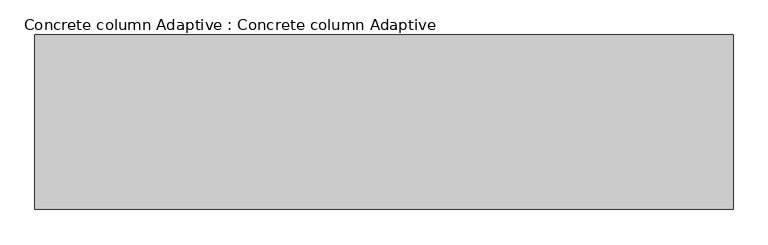
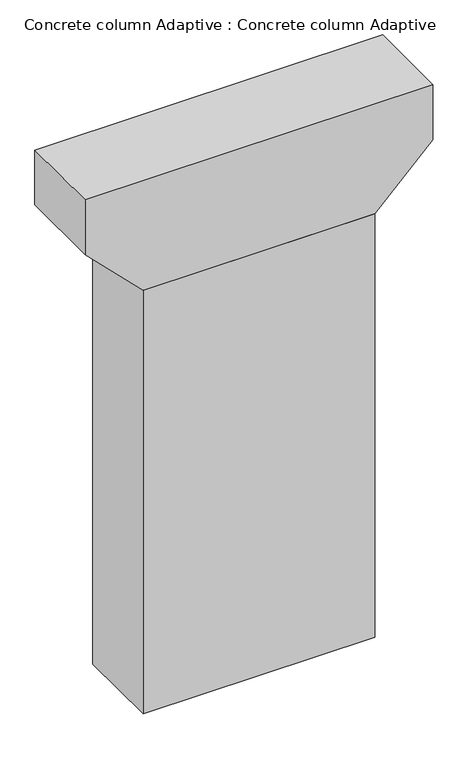
"""IFC4 building model written with IfcOpenShell, lengths in millimetres: proxy geometry, Concrete column Adaptive : Concrete column Adaptive."""

import ifcopenshell
import ifcopenshell.guid

model = None  # the IFC model being written
_history = None  # IfcOwnerHistory: only IFC2X3 demands one
_inside = {}  # id of a spatial element -> (the spatial element, [elements in it])
_under = {}  # id of a project, library or spatial element -> (it, [spatial elements below it])
_declared = {}  # id of a project -> (the project, [libraries it declares])
_typed = {}  # id of a type object -> (the type object, [elements of that type])
_made_of = {}  # id of a material, layer set ... -> (it, [elements and type objects made of it])


def new_model(schema):
    """Start an empty IFC model of exactly this schema.

    Asked for "IFC4X3", IfcOpenShell would pick the latest addendum, in which some entities
    have other attributes; the version numbers below select the first issue.
    IFC2X3 requires an IfcOwnerHistory on every rooted entity: one is made here for all.
    """
    global model, _history
    if schema == "IFC4X3":
        model = ifcopenshell.file(schema_version=(4, 3, 0, 0))
    else:
        model = ifcopenshell.file(schema=schema)
    _inside.clear()
    _under.clear()
    _declared.clear()
    _typed.clear()
    _made_of.clear()
    _history = None
    if model.schema == "IFC2X3":
        org = make("IfcOrganization", Name="unknown")
        user = make(
            "IfcPersonAndOrganization",
            ThePerson=make("IfcPerson", FamilyName="unknown"),
            TheOrganization=org,
        )
        app = make(
            "IfcApplication",
            ApplicationDeveloper=org,
            Version="unknown",
            ApplicationFullName="unknown",
            ApplicationIdentifier="unknown",
        )
        _history = make(
            "IfcOwnerHistory",
            OwningUser=user,
            OwningApplication=app,
            ChangeAction="ADDED",
            CreationDate=0,
        )
    return model


def make(cls, **values):
    """One entity of the class cls with the attributes given. An attribute that is None is left unset."""
    return model.create_entity(
        cls, **{name: value for name, value in values.items() if value is not None}
    )


def rooted(cls, **values):
    """An entity with a GlobalId (a new one), such as an element, a storey or a relation."""
    return make(cls, GlobalId=ifcopenshell.guid.new(), OwnerHistory=_history, **values)


def si_unit(unit_type, name, prefix=None):
    """IfcSIUnit, for example si_unit("LENGTHUNIT", "METRE", prefix="MILLI")."""
    return make("IfcSIUnit", UnitType=unit_type, Prefix=prefix, Name=name)


def assignment(units):
    """IfcUnitAssignment: the units of a project."""
    return None if units is None else make("IfcUnitAssignment", Units=units)


def point(xyz):
    """IfcCartesianPoint."""
    return None if xyz is None else make("IfcCartesianPoint", Coordinates=xyz)


def direction(xyz):
    """IfcDirection."""
    return None if xyz is None else make("IfcDirection", DirectionRatios=xyz)


def frame(location, z_axis=None, x_axis=None):
    """IfcAxis2Placement3D, a coordinate frame: its origin and axes. An axis left out is left unset."""
    return make(
        "IfcAxis2Placement3D",
        Location=point(location),
        Axis=direction(z_axis),
        RefDirection=direction(x_axis),
    )


def origin():
    """The frame at (0, 0, 0) with its axes left unset."""
    return frame((0.0, 0.0, 0.0))


def origin_with_axes():
    """The frame at (0, 0, 0) with the z axis (0, 0, 1) and the x axis (1, 0, 0) written out."""
    return frame((0.0, 0.0, 0.0), z_axis=(0.0, 0.0, 1.0), x_axis=(1.0, 0.0, 0.0))


def place(relative_to, where):
    """IfcLocalPlacement: puts the frame where relative to a parent placement (None: the world)."""
    return make(
        "IfcLocalPlacement", PlacementRelTo=relative_to, RelativePlacement=where
    )


def context(
    kind, dimensions, precision=None, world=None, true_north=None, identifier=None
):
    """IfcGeometricRepresentationContext, for example the 3D "Model" context."""
    return make(
        "IfcGeometricRepresentationContext",
        ContextIdentifier=identifier,
        ContextType=kind,
        CoordinateSpaceDimension=dimensions,
        Precision=precision,
        WorldCoordinateSystem=world,
        TrueNorth=true_north,
    )


def project(units=None, contexts=None):
    """IfcProject with its units and contexts."""
    return rooted(
        "IfcProject",
        Name="project",
        RepresentationContexts=contexts,
        UnitsInContext=assignment(units),
    )


def spatial(cls, under=None, at=None, **own):
    """A site, building, storey or space (cls), placed at a placement, below another one or the project."""
    s = rooted(cls, ObjectPlacement=at, **own)
    if under is not None:
        _under.setdefault(under.id(), (under, []))[1].append(s)
    return s


def polyline(points):
    """IfcPolyline through the points."""
    return make("IfcPolyline", Points=[point(p) for p in points])


def outline(outer, holes=None, kind="AREA"):
    """IfcArbitraryClosedProfileDef: a profile drawn as a closed curve; with holes, ...WithVoids."""
    if holes is None:
        return make("IfcArbitraryClosedProfileDef", ProfileType=kind, OuterCurve=outer)
    return make(
        "IfcArbitraryProfileDefWithVoids",
        ProfileType=kind,
        OuterCurve=outer,
        InnerCurves=holes,
    )


def extrude(swept, where, along, depth):
    """IfcExtrudedAreaSolid: the profile swept, set in the frame where, extruded along a direction by depth."""
    return make(
        "IfcExtrudedAreaSolid",
        SweptArea=swept,
        Position=where,
        ExtrudedDirection=direction(along),
        Depth=depth,
    )


def shape(context_of_items, identifier, shape_type, items):
    """IfcShapeRepresentation: the items that make up one representation, for example the "Body"."""
    return make(
        "IfcShapeRepresentation",
        ContextOfItems=context_of_items,
        RepresentationIdentifier=identifier,
        RepresentationType=shape_type,
        Items=items,
    )


def source(mapping_origin, context_of_items, identifier, shape_type, items):
    """IfcRepresentationMap: a shape defined once, which mapped items show again and again."""
    return make(
        "IfcRepresentationMap",
        MappingOrigin=mapping_origin,
        MappedRepresentation=shape(context_of_items, identifier, shape_type, items),
    )


def transform(
    local_origin,
    x_axis=None,
    y_axis=None,
    z_axis=None,
    scale=None,
    scale2=None,
    scale3=None,
    uniform=True,
):
    """IfcCartesianTransformationOperator3D, or its non-uniform kind. x_axis, y_axis, z_axis: its Axis1, 2, 3."""
    if uniform:
        return make(
            "IfcCartesianTransformationOperator3D",
            Axis1=direction(x_axis),
            Axis2=direction(y_axis),
            LocalOrigin=point(local_origin),
            Scale=scale,
            Axis3=direction(z_axis),
        )
    return make(
        "IfcCartesianTransformationOperator3DnonUniform",
        Axis1=direction(x_axis),
        Axis2=direction(y_axis),
        LocalOrigin=point(local_origin),
        Scale=scale,
        Axis3=direction(z_axis),
        Scale2=scale2,
        Scale3=scale3,
    )


def mapped(mapping_source, mapping_target):
    """IfcMappedItem: shows the shape of a source again, moved by a transform."""
    return make(
        "IfcMappedItem", MappingSource=mapping_source, MappingTarget=mapping_target
    )


def made_of(thing, what):
    """Note that an element or type object is made of a material, layer set ...; save() writes the relation."""
    if what is not None:
        _made_of.setdefault(what.id(), (what, []))[1].append(thing)
    return thing


def element(
    cls,
    number,
    at=None,
    inside=None,
    cuts=None,
    type_object=None,
    material=None,
    context=None,
    identifier="Body",
    shape_type=None,
    held_by="IfcProductDefinitionShape",
    body=None,
    shapes=None,
    **own,
):
    """One element of the class cls, such as IfcWall. Its Tag is "e" and its number.

    at: its placement. inside: the storey or other place that contains it. cuts: it is an
    opening in that element (IfcRelVoidsElement). A single representation is given by context,
    identifier, shape_type and body (its items); several are given by shapes. held_by: the class
    of the entity that holds the representations. save() writes the other relations.
    """
    e = rooted(cls, Tag="e%d" % number, ObjectPlacement=at, **own)
    if body is not None:
        shapes = [shape(context, identifier, shape_type, body)]
    if shapes is not None:
        e.Representation = make(held_by, Representations=shapes)
    if inside is not None:
        _inside.setdefault(inside.id(), (inside, []))[1].append(e)
    if cuts is not None:
        rooted(
            "IfcRelVoidsElement", RelatingBuildingElement=cuts, RelatedOpeningElement=e
        )
    if type_object is not None:
        _typed.setdefault(type_object.id(), (type_object, []))[1].append(e)
    return made_of(e, material)


def aggregate(whole, parts):
    """IfcRelAggregates: a whole, such as a stair, and the parts it consists of."""
    return rooted("IfcRelAggregates", RelatingObject=whole, RelatedObjects=parts)


def save(model, path):
    """Write the relations noted so far, then the file.

    IfcRelAggregates (storeys below a building ...), IfcRelContainedInSpatialStructure (elements
    in a storey), IfcRelDefinesByType, IfcRelAssociatesMaterial and IfcRelDeclares: one each for
    every whole, place, type object, material and project.
    """
    for whole, parts in _under.values():
        aggregate(whole, parts)
    for where, things in _inside.values():
        rooted(
            "IfcRelContainedInSpatialStructure",
            RelatedElements=things,
            RelatingStructure=where,
        )
    for kind, things in _typed.values():
        rooted("IfcRelDefinesByType", RelatedObjects=things, RelatingType=kind)
    for what, things in _made_of.values():
        rooted("IfcRelAssociatesMaterial", RelatedObjects=things, RelatingMaterial=what)
    for by, libraries in _declared.values():
        rooted("IfcRelDeclares", RelatingContext=by, RelatedDefinitions=libraries)
    model.write(path)


def concrete_column_adaptive_concrete_column_adaptive_030e40f1(model_context):
    return source(origin(), model_context, "Body", "SweptSolid", [
        extrude(outline(polyline([(19446.0, 6000.0), (19446.0, -6000.0), (17446.0, -6000.0), (15446.0, -4000.0), (15446.0, 4000.0), (17446.0, 6000.0), (19446.0, 6000.0)])), frame((0.0, -1500.0, 0.0), z_axis=(0.0, 1.0, 0.0), x_axis=(0.0, 0.0, 1.0)), (0.0, 0.0, 1.0), 3000.0),
        extrude(outline(polyline([(-4000.0, -1500.0), (-4000.0, 1500.0), (4000.0, 1500.0), (4000.0, -1500.0), (-4000.0, -1500.0)])), origin_with_axes(), (0.0, 0.0, 1.0), 15446.0),
    ])


if __name__ == "__main__":
    model = new_model("IFC4")
    model_context = context("Model", 3, world=origin())
    ifc_project = project(units=[si_unit("LENGTHUNIT", "METRE", prefix="MILLI")], contexts=[model_context])
    site = spatial("IfcSite", under=ifc_project)
    building = spatial("IfcBuilding", under=site)
    placement = place(None, origin())
    concrete_column_adaptive_concrete_column_adaptive_shape = concrete_column_adaptive_concrete_column_adaptive_030e40f1(model_context)
    element("IfcBuildingElementProxy", 1, Name="Concrete column Adaptive : Concrete column Adaptive", ObjectType="Concrete column Adaptive : Concrete column Adaptive", at=placement, inside=building, context=model_context, shape_type="MappedRepresentation", body=[
        mapped(concrete_column_adaptive_concrete_column_adaptive_shape, transform((0.0, 0.0, 0.0), x_axis=(1.0, 0.0, 0.0), y_axis=(0.0, 1.0, 0.0), z_axis=(0.0, 0.0, 1.0))),
    ])
    save(model, "model.ifc")

# Revit data of these elements
# Project information
#   Project Issue Date = "Issue Date"
#   Project Status = "Project Status"
#   Client Name = "Owner"
#   Project Address = "Enter address here"
#   Project Name = "Project Name"
#   Project Number = "Project Number"
# Type "Concrete column Adaptive : Concrete column Adaptive"
#   Height [instance default] = 30000 mm
#   Default Elevation = 0
# Element 1 (IfcBuildingElementProxy, "Concrete column Adaptive : Concrete column Adaptive")
#   Height = 15446 mm
#   Materials on its faces: "Default Wall"
# Materials
#   "Default Wall": class "Miscellaneous", colour RGB 128 128 128, transparency 0, Comments = "Rendering appearance not upgraded Rendering appearance not upgraded ", Cost = 0
